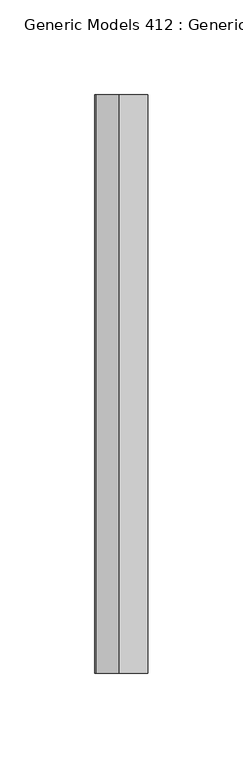
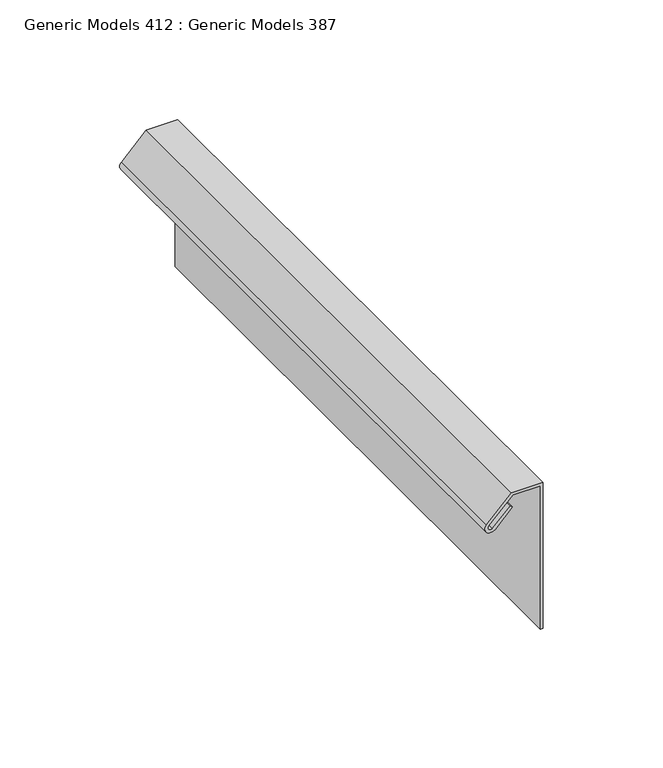
"""IFC4 building model written with IfcOpenShell, lengths in millimetres: proxy geometry, Generic Models 412 : Generic Models 387."""

import ifcopenshell
import ifcopenshell.guid

model = None  # the IFC model being written
_history = None  # IfcOwnerHistory: only IFC2X3 demands one
_inside = {}  # id of a spatial element -> (the spatial element, [elements in it])
_under = {}  # id of a project, library or spatial element -> (it, [spatial elements below it])
_declared = {}  # id of a project -> (the project, [libraries it declares])
_typed = {}  # id of a type object -> (the type object, [elements of that type])
_made_of = {}  # id of a material, layer set ... -> (it, [elements and type objects made of it])


def new_model(schema):
    """Start an empty IFC model of exactly this schema.

    Asked for "IFC4X3", IfcOpenShell would pick the latest addendum, in which some entities
    have other attributes; the version numbers below select the first issue.
    IFC2X3 requires an IfcOwnerHistory on every rooted entity: one is made here for all.
    """
    global model, _history
    if schema == "IFC4X3":
        model = ifcopenshell.file(schema_version=(4, 3, 0, 0))
    else:
        model = ifcopenshell.file(schema=schema)
    _inside.clear()
    _under.clear()
    _declared.clear()
    _typed.clear()
    _made_of.clear()
    _history = None
    if model.schema == "IFC2X3":
        org = make("IfcOrganization", Name="unknown")
        user = make(
            "IfcPersonAndOrganization",
            ThePerson=make("IfcPerson", FamilyName="unknown"),
            TheOrganization=org,
        )
        app = make(
            "IfcApplication",
            ApplicationDeveloper=org,
            Version="unknown",
            ApplicationFullName="unknown",
            ApplicationIdentifier="unknown",
        )
        _history = make(
            "IfcOwnerHistory",
            OwningUser=user,
            OwningApplication=app,
            ChangeAction="ADDED",
            CreationDate=0,
        )
    return model


def make(cls, **values):
    """One entity of the class cls with the attributes given. An attribute that is None is left unset."""
    return model.create_entity(
        cls, **{name: value for name, value in values.items() if value is not None}
    )


def rooted(cls, **values):
    """An entity with a GlobalId (a new one), such as an element, a storey or a relation."""
    return make(cls, GlobalId=ifcopenshell.guid.new(), OwnerHistory=_history, **values)


def si_unit(unit_type, name, prefix=None):
    """IfcSIUnit, for example si_unit("LENGTHUNIT", "METRE", prefix="MILLI")."""
    return make("IfcSIUnit", UnitType=unit_type, Prefix=prefix, Name=name)


def assignment(units):
    """IfcUnitAssignment: the units of a project."""
    return None if units is None else make("IfcUnitAssignment", Units=units)


def point(xyz):
    """IfcCartesianPoint."""
    return None if xyz is None else make("IfcCartesianPoint", Coordinates=xyz)


def direction(xyz):
    """IfcDirection."""
    return None if xyz is None else make("IfcDirection", DirectionRatios=xyz)


def frame(location, z_axis=None, x_axis=None):
    """IfcAxis2Placement3D, a coordinate frame: its origin and axes. An axis left out is left unset."""
    return make(
        "IfcAxis2Placement3D",
        Location=point(location),
        Axis=direction(z_axis),
        RefDirection=direction(x_axis),
    )


def frame_2d(location, x_axis=None):
    """IfcAxis2Placement2D, a coordinate frame in the plane: its origin and x axis."""
    return make(
        "IfcAxis2Placement2D", Location=point(location), RefDirection=direction(x_axis)
    )


def origin():
    """The frame at (0, 0, 0) with its axes left unset."""
    return frame((0.0, 0.0, 0.0))


def place(relative_to, where):
    """IfcLocalPlacement: puts the frame where relative to a parent placement (None: the world)."""
    return make(
        "IfcLocalPlacement", PlacementRelTo=relative_to, RelativePlacement=where
    )


def context(
    kind, dimensions, precision=None, world=None, true_north=None, identifier=None
):
    """IfcGeometricRepresentationContext, for example the 3D "Model" context."""
    return make(
        "IfcGeometricRepresentationContext",
        ContextIdentifier=identifier,
        ContextType=kind,
        CoordinateSpaceDimension=dimensions,
        Precision=precision,
        WorldCoordinateSystem=world,
        TrueNorth=true_north,
    )


def project(units=None, contexts=None):
    """IfcProject with its units and contexts."""
    return rooted(
        "IfcProject",
        Name="project",
        RepresentationContexts=contexts,
        UnitsInContext=assignment(units),
    )


def spatial(cls, under=None, at=None, **own):
    """A site, building, storey or space (cls), placed at a placement, below another one or the project."""
    s = rooted(cls, ObjectPlacement=at, **own)
    if under is not None:
        _under.setdefault(under.id(), (under, []))[1].append(s)
    return s


def polyline(points):
    """IfcPolyline through the points."""
    return make("IfcPolyline", Points=[point(p) for p in points])


def circle_curve(where, radius):
    """IfcCircle in the frame where."""
    return make("IfcCircle", Position=where, Radius=radius)


def trimmed(basis, trim1, trim2, sense, master):
    """IfcTrimmedCurve: the piece of a basis curve between two trims."""
    return make(
        "IfcTrimmedCurve",
        BasisCurve=basis,
        Trim1=trim1,
        Trim2=trim2,
        SenseAgreement=sense,
        MasterRepresentation=master,
    )


def segment(curve, same_sense, transition):
    """IfcCompositeCurveSegment."""
    return make(
        "IfcCompositeCurveSegment",
        Transition=transition,
        SameSense=same_sense,
        ParentCurve=curve,
    )


def composite_curve(segments, self_intersect=None):
    """IfcCompositeCurve: segments joined end to end."""
    return make("IfcCompositeCurve", Segments=segments, SelfIntersect=self_intersect)


def outline(outer, holes=None, kind="AREA"):
    """IfcArbitraryClosedProfileDef: a profile drawn as a closed curve; with holes, ...WithVoids."""
    if holes is None:
        return make("IfcArbitraryClosedProfileDef", ProfileType=kind, OuterCurve=outer)
    return make(
        "IfcArbitraryProfileDefWithVoids",
        ProfileType=kind,
        OuterCurve=outer,
        InnerCurves=holes,
    )


def extrude(swept, where, along, depth):
    """IfcExtrudedAreaSolid: the profile swept, set in the frame where, extruded along a direction by depth."""
    return make(
        "IfcExtrudedAreaSolid",
        SweptArea=swept,
        Position=where,
        ExtrudedDirection=direction(along),
        Depth=depth,
    )


def shape(context_of_items, identifier, shape_type, items):
    """IfcShapeRepresentation: the items that make up one representation, for example the "Body"."""
    return make(
        "IfcShapeRepresentation",
        ContextOfItems=context_of_items,
        RepresentationIdentifier=identifier,
        RepresentationType=shape_type,
        Items=items,
    )


def source(mapping_origin, context_of_items, identifier, shape_type, items):
    """IfcRepresentationMap: a shape defined once, which mapped items show again and again."""
    return make(
        "IfcRepresentationMap",
        MappingOrigin=mapping_origin,
        MappedRepresentation=shape(context_of_items, identifier, shape_type, items),
    )


def transform(
    local_origin,
    x_axis=None,
    y_axis=None,
    z_axis=None,
    scale=None,
    scale2=None,
    scale3=None,
    uniform=True,
):
    """IfcCartesianTransformationOperator3D, or its non-uniform kind. x_axis, y_axis, z_axis: its Axis1, 2, 3."""
    if uniform:
        return make(
            "IfcCartesianTransformationOperator3D",
            Axis1=direction(x_axis),
            Axis2=direction(y_axis),
            LocalOrigin=point(local_origin),
            Scale=scale,
            Axis3=direction(z_axis),
        )
    return make(
        "IfcCartesianTransformationOperator3DnonUniform",
        Axis1=direction(x_axis),
        Axis2=direction(y_axis),
        LocalOrigin=point(local_origin),
        Scale=scale,
        Axis3=direction(z_axis),
        Scale2=scale2,
        Scale3=scale3,
    )


def mapped(mapping_source, mapping_target):
    """IfcMappedItem: shows the shape of a source again, moved by a transform."""
    return make(
        "IfcMappedItem", MappingSource=mapping_source, MappingTarget=mapping_target
    )


def made_of(thing, what):
    """Note that an element or type object is made of a material, layer set ...; save() writes the relation."""
    if what is not None:
        _made_of.setdefault(what.id(), (what, []))[1].append(thing)
    return thing


def element(
    cls,
    number,
    at=None,
    inside=None,
    cuts=None,
    type_object=None,
    material=None,
    context=None,
    identifier="Body",
    shape_type=None,
    held_by="IfcProductDefinitionShape",
    body=None,
    shapes=None,
    **own,
):
    """One element of the class cls, such as IfcWall. Its Tag is "e" and its number.

    at: its placement. inside: the storey or other place that contains it. cuts: it is an
    opening in that element (IfcRelVoidsElement). A single representation is given by context,
    identifier, shape_type and body (its items); several are given by shapes. held_by: the class
    of the entity that holds the representations. save() writes the other relations.
    """
    e = rooted(cls, Tag="e%d" % number, ObjectPlacement=at, **own)
    if body is not None:
        shapes = [shape(context, identifier, shape_type, body)]
    if shapes is not None:
        e.Representation = make(held_by, Representations=shapes)
    if inside is not None:
        _inside.setdefault(inside.id(), (inside, []))[1].append(e)
    if cuts is not None:
        rooted(
            "IfcRelVoidsElement", RelatingBuildingElement=cuts, RelatedOpeningElement=e
        )
    if type_object is not None:
        _typed.setdefault(type_object.id(), (type_object, []))[1].append(e)
    return made_of(e, material)


def aggregate(whole, parts):
    """IfcRelAggregates: a whole, such as a stair, and the parts it consists of."""
    return rooted("IfcRelAggregates", RelatingObject=whole, RelatedObjects=parts)


def save(model, path):
    """Write the relations noted so far, then the file.

    IfcRelAggregates (storeys below a building ...), IfcRelContainedInSpatialStructure (elements
    in a storey), IfcRelDefinesByType, IfcRelAssociatesMaterial and IfcRelDeclares: one each for
    every whole, place, type object, material and project.
    """
    for whole, parts in _under.values():
        aggregate(whole, parts)
    for where, things in _inside.values():
        rooted(
            "IfcRelContainedInSpatialStructure",
            RelatedElements=things,
            RelatingStructure=where,
        )
    for kind, things in _typed.values():
        rooted("IfcRelDefinesByType", RelatedObjects=things, RelatingType=kind)
    for what, things in _made_of.values():
        rooted("IfcRelAssociatesMaterial", RelatedObjects=things, RelatingMaterial=what)
    for by, libraries in _declared.values():
        rooted("IfcRelDeclares", RelatingContext=by, RelatedDefinitions=libraries)
    model.write(path)


def generic_models_412_generic_models_387_579364b1(model_context):
    return source(origin(), model_context, "Body", "SweptSolid", [
        extrude(outline(composite_curve([segment(polyline([(127264.3289779, -7051.7971429), (127338.7321716, -7051.7971429), (127338.7321716, -7067.0009179), (127326.7506172, -7078.9824723)]), True, "CONTINUOUS"), segment(trimmed(circle_curve(frame_2d((127324.7895938, -7077.0214489)), 2.7733058), [point((127326.7506172, -7078.9824723))], [point((127322.8285705, -7075.0604255))], False, "CARTESIAN"), True, "CONTINUOUS"), segment(polyline([(127322.8285705, -7075.0604255), (127331.4088985, -7066.4800975), (127332.3959826, -7067.4671816), (127323.8156546, -7076.0475096)]), True, "CONTINUOUS"), segment(trimmed(circle_curve(frame_2d((127324.7895938, -7077.0214489)), 1.3773581), [point((127323.8156546, -7076.0475096))], [point((127325.7452461, -7078.0133381))], True, "CARTESIAN"), True, "CONTINUOUS"), segment(polyline([(127325.7452461, -7078.0133381), (127337.4423279, -7066.3162563), (127337.4423279, -7053.0869866), (127264.3289779, -7053.0869866), (127264.3289779, -7051.7971429)]), True, "CONTINUOUS")], self_intersect=False)), frame((0.0, -4250.542257, 0.0), z_axis=(0.0, 1.0, 0.0), x_axis=(0.0, 0.0, 1.0)), (0.0, 0.0, 1.0), 304.8),
    ])


if __name__ == "__main__":
    model = new_model("IFC4")
    model_context = context("Model", 3, world=origin())
    ifc_project = project(units=[si_unit("LENGTHUNIT", "METRE", prefix="MILLI")], contexts=[model_context])
    site = spatial("IfcSite", under=ifc_project)
    building = spatial("IfcBuilding", under=site)
    placement = place(None, origin())
    generic_models_412_generic_models_387_shape = generic_models_412_generic_models_387_579364b1(model_context)
    element("IfcBuildingElementProxy", 1, Name="Generic Models 412 : Generic Models 387", ObjectType="Generic Models 412 : Generic Models 387", at=placement, inside=building, context=model_context, shape_type="MappedRepresentation", body=[
        mapped(generic_models_412_generic_models_387_shape, transform((0.0, 0.0, 0.0), x_axis=(1.0, 0.0, 0.0), y_axis=(0.0, 1.0, 0.0), z_axis=(0.0, 0.0, 1.0))),
    ])
    save(model, "model.ifc")

# Revit data of these elements
# Element 1 (IfcBuildingElementProxy, "Generic Models 412 : Generic Models 387")
#   Materials on its faces: "_CONT. 16 GA. COPPER DRIP FLASHING"
# Materials
#   "_CONT. 16 GA. COPPER DRIP FLASHING": class "Metal", colour RGB 199 199 199, transparency 0, Description = "Structural steel 50ksi", Cost = 0
